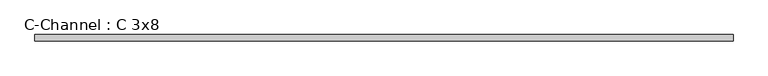
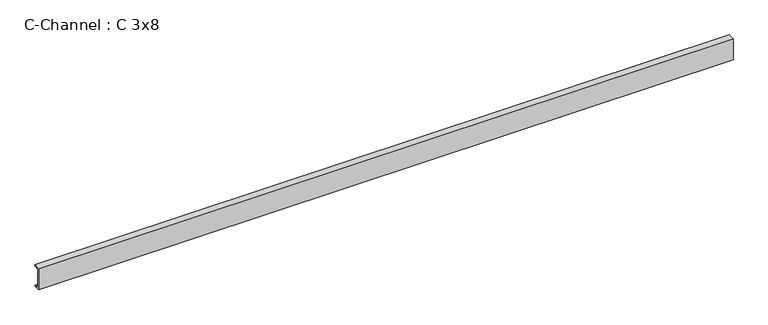
"""IFC4 building model written with IfcOpenShell, lengths in millimetres: beam geometry, C-Channel : C 3x8."""

import ifcopenshell
import ifcopenshell.guid

model = None  # the IFC model being written
_history = None  # IfcOwnerHistory: only IFC2X3 demands one
_inside = {}  # id of a spatial element -> (the spatial element, [elements in it])
_under = {}  # id of a project, library or spatial element -> (it, [spatial elements below it])
_declared = {}  # id of a project -> (the project, [libraries it declares])
_typed = {}  # id of a type object -> (the type object, [elements of that type])
_made_of = {}  # id of a material, layer set ... -> (it, [elements and type objects made of it])


def new_model(schema):
    """Start an empty IFC model of exactly this schema.

    Asked for "IFC4X3", IfcOpenShell would pick the latest addendum, in which some entities
    have other attributes; the version numbers below select the first issue.
    IFC2X3 requires an IfcOwnerHistory on every rooted entity: one is made here for all.
    """
    global model, _history
    if schema == "IFC4X3":
        model = ifcopenshell.file(schema_version=(4, 3, 0, 0))
    else:
        model = ifcopenshell.file(schema=schema)
    _inside.clear()
    _under.clear()
    _declared.clear()
    _typed.clear()
    _made_of.clear()
    _history = None
    if model.schema == "IFC2X3":
        org = make("IfcOrganization", Name="unknown")
        user = make(
            "IfcPersonAndOrganization",
            ThePerson=make("IfcPerson", FamilyName="unknown"),
            TheOrganization=org,
        )
        app = make(
            "IfcApplication",
            ApplicationDeveloper=org,
            Version="unknown",
            ApplicationFullName="unknown",
            ApplicationIdentifier="unknown",
        )
        _history = make(
            "IfcOwnerHistory",
            OwningUser=user,
            OwningApplication=app,
            ChangeAction="ADDED",
            CreationDate=0,
        )
    return model


def make(cls, **values):
    """One entity of the class cls with the attributes given. An attribute that is None is left unset."""
    return model.create_entity(
        cls, **{name: value for name, value in values.items() if value is not None}
    )


def rooted(cls, **values):
    """An entity with a GlobalId (a new one), such as an element, a storey or a relation."""
    return make(cls, GlobalId=ifcopenshell.guid.new(), OwnerHistory=_history, **values)


def si_unit(unit_type, name, prefix=None):
    """IfcSIUnit, for example si_unit("LENGTHUNIT", "METRE", prefix="MILLI")."""
    return make("IfcSIUnit", UnitType=unit_type, Prefix=prefix, Name=name)


def assignment(units):
    """IfcUnitAssignment: the units of a project."""
    return None if units is None else make("IfcUnitAssignment", Units=units)


def point(xyz):
    """IfcCartesianPoint."""
    return None if xyz is None else make("IfcCartesianPoint", Coordinates=xyz)


def direction(xyz):
    """IfcDirection."""
    return None if xyz is None else make("IfcDirection", DirectionRatios=xyz)


def frame(location, z_axis=None, x_axis=None):
    """IfcAxis2Placement3D, a coordinate frame: its origin and axes. An axis left out is left unset."""
    return make(
        "IfcAxis2Placement3D",
        Location=point(location),
        Axis=direction(z_axis),
        RefDirection=direction(x_axis),
    )


def frame_2d(location, x_axis=None):
    """IfcAxis2Placement2D, a coordinate frame in the plane: its origin and x axis."""
    return make(
        "IfcAxis2Placement2D", Location=point(location), RefDirection=direction(x_axis)
    )


def origin():
    """The frame at (0, 0, 0) with its axes left unset."""
    return frame((0.0, 0.0, 0.0))


def place(relative_to, where):
    """IfcLocalPlacement: puts the frame where relative to a parent placement (None: the world)."""
    return make(
        "IfcLocalPlacement", PlacementRelTo=relative_to, RelativePlacement=where
    )


def context(
    kind, dimensions, precision=None, world=None, true_north=None, identifier=None
):
    """IfcGeometricRepresentationContext, for example the 3D "Model" context."""
    return make(
        "IfcGeometricRepresentationContext",
        ContextIdentifier=identifier,
        ContextType=kind,
        CoordinateSpaceDimension=dimensions,
        Precision=precision,
        WorldCoordinateSystem=world,
        TrueNorth=true_north,
    )


def project(units=None, contexts=None):
    """IfcProject with its units and contexts."""
    return rooted(
        "IfcProject",
        Name="project",
        RepresentationContexts=contexts,
        UnitsInContext=assignment(units),
    )


def spatial(cls, under=None, at=None, **own):
    """A site, building, storey or space (cls), placed at a placement, below another one or the project."""
    s = rooted(cls, ObjectPlacement=at, **own)
    if under is not None:
        _under.setdefault(under.id(), (under, []))[1].append(s)
    return s


def polyline(points):
    """IfcPolyline through the points."""
    return make("IfcPolyline", Points=[point(p) for p in points])


def circle_curve(where, radius):
    """IfcCircle in the frame where."""
    return make("IfcCircle", Position=where, Radius=radius)


def trimmed(basis, trim1, trim2, sense, master):
    """IfcTrimmedCurve: the piece of a basis curve between two trims."""
    return make(
        "IfcTrimmedCurve",
        BasisCurve=basis,
        Trim1=trim1,
        Trim2=trim2,
        SenseAgreement=sense,
        MasterRepresentation=master,
    )


def segment(curve, same_sense, transition):
    """IfcCompositeCurveSegment."""
    return make(
        "IfcCompositeCurveSegment",
        Transition=transition,
        SameSense=same_sense,
        ParentCurve=curve,
    )


def composite_curve(segments, self_intersect=None):
    """IfcCompositeCurve: segments joined end to end."""
    return make("IfcCompositeCurve", Segments=segments, SelfIntersect=self_intersect)


def outline(outer, holes=None, kind="AREA"):
    """IfcArbitraryClosedProfileDef: a profile drawn as a closed curve; with holes, ...WithVoids."""
    if holes is None:
        return make("IfcArbitraryClosedProfileDef", ProfileType=kind, OuterCurve=outer)
    return make(
        "IfcArbitraryProfileDefWithVoids",
        ProfileType=kind,
        OuterCurve=outer,
        InnerCurves=holes,
    )


def extrude(swept, where, along, depth):
    """IfcExtrudedAreaSolid: the profile swept, set in the frame where, extruded along a direction by depth."""
    return make(
        "IfcExtrudedAreaSolid",
        SweptArea=swept,
        Position=where,
        ExtrudedDirection=direction(along),
        Depth=depth,
    )


def shape(context_of_items, identifier, shape_type, items):
    """IfcShapeRepresentation: the items that make up one representation, for example the "Body"."""
    return make(
        "IfcShapeRepresentation",
        ContextOfItems=context_of_items,
        RepresentationIdentifier=identifier,
        RepresentationType=shape_type,
        Items=items,
    )


def source(mapping_origin, context_of_items, identifier, shape_type, items):
    """IfcRepresentationMap: a shape defined once, which mapped items show again and again."""
    return make(
        "IfcRepresentationMap",
        MappingOrigin=mapping_origin,
        MappedRepresentation=shape(context_of_items, identifier, shape_type, items),
    )


def transform(
    local_origin,
    x_axis=None,
    y_axis=None,
    z_axis=None,
    scale=None,
    scale2=None,
    scale3=None,
    uniform=True,
):
    """IfcCartesianTransformationOperator3D, or its non-uniform kind. x_axis, y_axis, z_axis: its Axis1, 2, 3."""
    if uniform:
        return make(
            "IfcCartesianTransformationOperator3D",
            Axis1=direction(x_axis),
            Axis2=direction(y_axis),
            LocalOrigin=point(local_origin),
            Scale=scale,
            Axis3=direction(z_axis),
        )
    return make(
        "IfcCartesianTransformationOperator3DnonUniform",
        Axis1=direction(x_axis),
        Axis2=direction(y_axis),
        LocalOrigin=point(local_origin),
        Scale=scale,
        Axis3=direction(z_axis),
        Scale2=scale2,
        Scale3=scale3,
    )


def mapped(mapping_source, mapping_target):
    """IfcMappedItem: shows the shape of a source again, moved by a transform."""
    return make(
        "IfcMappedItem", MappingSource=mapping_source, MappingTarget=mapping_target
    )


def made_of(thing, what):
    """Note that an element or type object is made of a material, layer set ...; save() writes the relation."""
    if what is not None:
        _made_of.setdefault(what.id(), (what, []))[1].append(thing)
    return thing


def element(
    cls,
    number,
    at=None,
    inside=None,
    cuts=None,
    type_object=None,
    material=None,
    context=None,
    identifier="Body",
    shape_type=None,
    held_by="IfcProductDefinitionShape",
    body=None,
    shapes=None,
    **own,
):
    """One element of the class cls, such as IfcWall. Its Tag is "e" and its number.

    at: its placement. inside: the storey or other place that contains it. cuts: it is an
    opening in that element (IfcRelVoidsElement). A single representation is given by context,
    identifier, shape_type and body (its items); several are given by shapes. held_by: the class
    of the entity that holds the representations. save() writes the other relations.
    """
    e = rooted(cls, Tag="e%d" % number, ObjectPlacement=at, **own)
    if body is not None:
        shapes = [shape(context, identifier, shape_type, body)]
    if shapes is not None:
        e.Representation = make(held_by, Representations=shapes)
    if inside is not None:
        _inside.setdefault(inside.id(), (inside, []))[1].append(e)
    if cuts is not None:
        rooted(
            "IfcRelVoidsElement", RelatingBuildingElement=cuts, RelatedOpeningElement=e
        )
    if type_object is not None:
        _typed.setdefault(type_object.id(), (type_object, []))[1].append(e)
    return made_of(e, material)


def aggregate(whole, parts):
    """IfcRelAggregates: a whole, such as a stair, and the parts it consists of."""
    return rooted("IfcRelAggregates", RelatingObject=whole, RelatedObjects=parts)


def save(model, path):
    """Write the relations noted so far, then the file.

    IfcRelAggregates (storeys below a building ...), IfcRelContainedInSpatialStructure (elements
    in a storey), IfcRelDefinesByType, IfcRelAssociatesMaterial and IfcRelDeclares: one each for
    every whole, place, type object, material and project.
    """
    for whole, parts in _under.values():
        aggregate(whole, parts)
    for where, things in _inside.values():
        rooted(
            "IfcRelContainedInSpatialStructure",
            RelatedElements=things,
            RelatingStructure=where,
        )
    for kind, things in _typed.values():
        rooted("IfcRelDefinesByType", RelatedObjects=things, RelatingType=kind)
    for what, things in _made_of.values():
        rooted("IfcRelAssociatesMaterial", RelatedObjects=things, RelatingMaterial=what)
    for by, libraries in _declared.values():
        rooted("IfcRelDeclares", RelatingContext=by, RelatedDefinitions=libraries)
    model.write(path)


def c_channel_c_3x8_649f6971(model_context):
    return source(origin(), model_context, "Body", "SweptSolid", [
        extrude(outline(composite_curve([segment(polyline([(-13.5128, 101.6), (44.9072, 101.6)]), True, "CONTINUOUS"), segment(trimmed(circle_curve(frame_2d((35.6108, 101.6)), 9.2964), [point((44.9072, 101.6))], [point((35.6108, 92.3036))], False, "CARTESIAN"), True, "CONTINUOUS"), segment(polyline([(35.6108, 92.3036), (-2.8702, 86.2088084), (-2.8702, -86.2088084), (35.6108, -92.3036)]), True, "CONTINUOUS"), segment(trimmed(circle_curve(frame_2d((35.6108, -101.6)), 9.2964), [point((35.6108, -92.3036))], [point((44.9072, -101.6))], False, "CARTESIAN"), True, "CONTINUOUS"), segment(polyline([(44.9072, -101.6), (-13.5128, -101.6), (-13.5128, 101.6)]), True, "CONTINUOUS")], self_intersect=False)), frame((-3168.65, 0.0, 0.0), z_axis=(1.0, 0.0, 0.0), x_axis=(0.0, 1.0, 0.0)), (0.0, 0.0, 1.0), 6337.3),
    ])


if __name__ == "__main__":
    model = new_model("IFC4")
    model_context = context("Model", 3, world=origin())
    ifc_project = project(units=[si_unit("LENGTHUNIT", "METRE", prefix="MILLI")], contexts=[model_context])
    site = spatial("IfcSite", under=ifc_project)
    building = spatial("IfcBuilding", under=site)
    placement = place(None, origin())
    c_channel_c_3x8_shape = c_channel_c_3x8_649f6971(model_context)
    element("IfcBeam", 1, ObjectType="C-Channel : C 3x8", at=placement, inside=building, context=model_context, shape_type="MappedRepresentation", body=[
        mapped(c_channel_c_3x8_shape, transform((0.0, 0.0, 0.0), x_axis=(1.0, 0.0, 0.0), y_axis=(0.0, 1.0, 0.0), z_axis=(0.0, 0.0, 1.0))),
    ])
    save(model, "model.ifc")

# Revit data of these elements
# Type "C-Channel : C 3x8"
#   Assembly Code = "B10"
#   W = 14.7
#   Length [instance default] = 5' - 0"
#   bf = 0' - 2.3"
#   d = 0' - 8"
#   tf = 0' - 0.366"
#   tw = 0' - 0.419"
#   x = 0' - 0.532"
#   A = 0.0300694 SF
#   Structural Material [instance default] = Steel ASTM A36
# Element 1 (IfcBeam, "C-Channel : C 3x8")
#   Structural Material = Steel ASTM A992
#   Materials on its faces: "Steel ASTM A992"
# Materials
#   "Steel ASTM A36": class "Metal", colour RGB 199 199 199, transparency 0, Description = "Structural steel, ASTM A36 Grade B, mill finish", Cost = 0
#   "Steel ASTM A992": class "Metal", colour RGB 189 187 185, transparency 0, Description = "Structural steel 50ksi", Cost = 0
